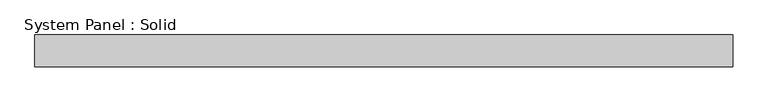
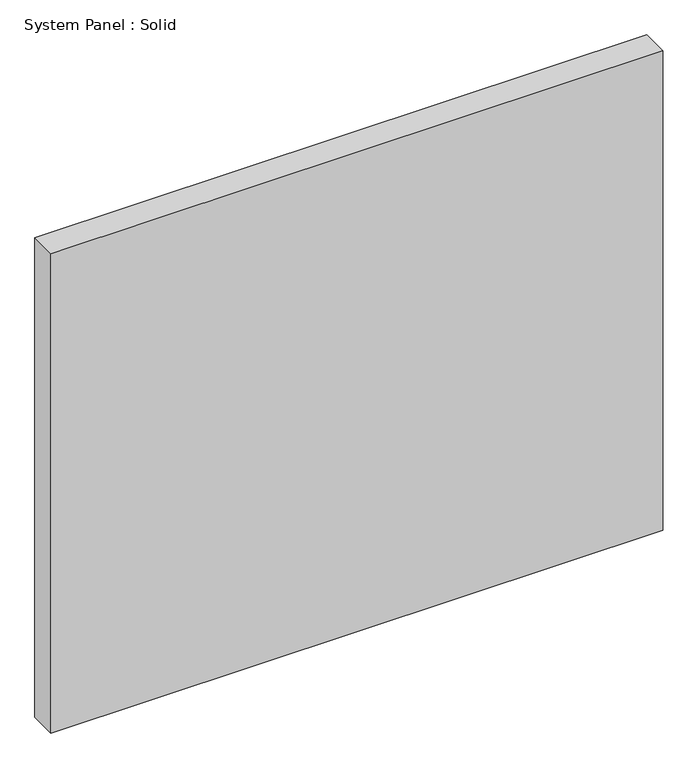
"""IFC4 building model written with IfcOpenShell, lengths in millimetres: plate geometry, System Panel : Solid."""

from ifc_helpers import new_model, si_unit, origin, origin_with_axes, place, context, project, spatial, polyline, outline, extrude, source, transform, mapped, element, save


def system_panel_solid_8f383511(model_context):
    return source(origin(), model_context, "Body", "SweptSolid", [
        extrude(outline(polyline([(697.4416668, -19.05), (-697.4416668, -19.05), (-697.4416668, 44.45), (697.4416668, 44.45), (697.4416668, -19.05)])), origin_with_axes(), (0.0, 0.0, 1.0), 1155.7),
    ])


if __name__ == "__main__":
    model = new_model("IFC4")
    model_context = context("Model", 3, world=origin())
    ifc_project = project(units=[si_unit("LENGTHUNIT", "METRE", prefix="MILLI")], contexts=[model_context])
    site = spatial("IfcSite", under=ifc_project)
    building = spatial("IfcBuilding", under=site)
    placement = place(None, origin())
    system_panel_solid_shape = system_panel_solid_8f383511(model_context)
    element("IfcPlate", 1, ObjectType="System Panel : Solid", at=placement, inside=building, context=model_context, shape_type="MappedRepresentation", body=[
        mapped(system_panel_solid_shape, transform((0.0, 0.0, 0.0), x_axis=(1.0, 0.0, 0.0), y_axis=(0.0, 1.0, 0.0), z_axis=(0.0, 0.0, 1.0))),
    ])
    save(model, "model.ifc")

# Revit data of these elements
# Type "System Panel : Solid"
#   Construction Type Id = "MDOOR"
#   Analytic Construction = "Metal"
#   Visual Light Transmittance = 0
#   Solar Heat Gain Coefficient = 0
#   Heat Transfer Coefficient (U) = 0.651978 BTU/(h·ft²·°F)
#   Define Thermal Properties by = 1
# Element 1 (IfcPlate, "System Panel : Solid")
#   Materials on its faces: "Default"
# Materials
#   "Default": class "Miscellaneous", colour RGB 127 127 127, transparency 0, Cost = 0
